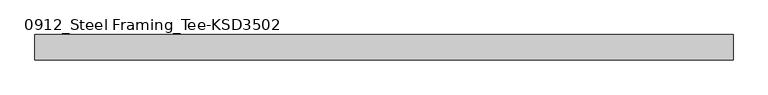
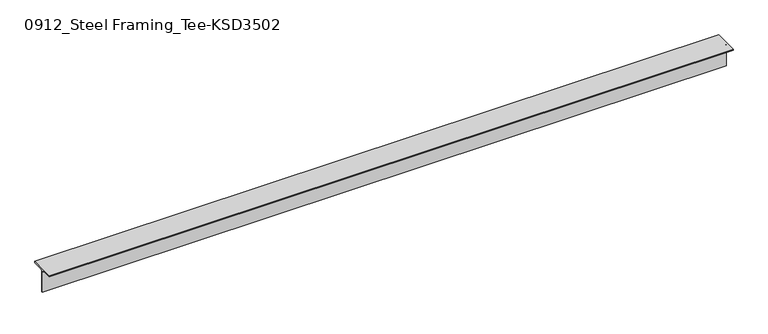
"""IFC4 building model written with IfcOpenShell, lengths in millimetres: member geometry, 0912_Steel Framing_Tee-KSD3502 : H_SB_ASB_CT-150x150x6.5x9."""

from ifc_helpers import new_model, si_unit, point, frame, frame_2d, origin, place, context, project, spatial, polyline, circle_curve, trimmed, segment, composite_curve, outline, extrude, source, transform, mapped, element, save


def member_0912_steel_framing_tee_ksd3502_90e65c15(model_context):
    return source(origin(), model_context, "Body", "SweptSolid", [
        extrude(outline(composite_curve([segment(polyline([(-75.0, 75.0), (75.0, 75.0), (75.0, 66.0), (16.25, 66.0)]), True, "CONTINUOUS"), segment(trimmed(circle_curve(frame_2d((16.25, 53.0)), 13.0), [point((16.25, 66.0))], [point((3.25, 53.0))], True, "CARTESIAN"), True, "CONTINUOUS"), segment(polyline([(3.25, 53.0), (3.25, -75.0), (-3.25, -75.0), (-3.25, 53.0)]), True, "CONTINUOUS"), segment(trimmed(circle_curve(frame_2d((-16.25, 53.0)), 13.0), [point((-3.25, 53.0))], [point((-16.25, 66.0))], True, "CARTESIAN"), True, "CONTINUOUS"), segment(polyline([(-16.25, 66.0), (-75.0, 66.0), (-75.0, 75.0)]), True, "CONTINUOUS")], self_intersect=False)), frame((-2093.8, 0.0, 0.0), z_axis=(1.0, 0.0, 0.0), x_axis=(0.0, 1.0, 0.0)), (0.0, 0.0, 1.0), 4153.3),
    ])


if __name__ == "__main__":
    model = new_model("IFC4")
    model_context = context("Model", 3, world=origin())
    ifc_project = project(units=[si_unit("LENGTHUNIT", "METRE", prefix="MILLI")], contexts=[model_context])
    site = spatial("IfcSite", under=ifc_project)
    building = spatial("IfcBuilding", under=site)
    placement = place(None, origin())
    member_0912_steel_framing_tee_ksd3502_shape = member_0912_steel_framing_tee_ksd3502_90e65c15(model_context)
    element("IfcMember", 1, ObjectType="0912_Steel Framing_Tee-KSD3502 : H_SB_ASB_CT-150x150x6.5x9", at=placement, inside=building, context=model_context, shape_type="MappedRepresentation", body=[
        mapped(member_0912_steel_framing_tee_ksd3502_shape, transform((0.0, 0.0, 0.0), x_axis=(1.0, 0.0, 0.0), y_axis=(0.0, 1.0, 0.0), z_axis=(0.0, 0.0, 1.0))),
    ])
    save(model, "model.ifc")

# Revit data of these elements
# Type "0912_Steel Framing_Tee-KSD3502 : H_SB_ASB_CT-150x150x6.5x9"
#   H_WM Code_1 = "S01AA003-00001 | Main Steel Structure Fabrication Work | Shelter/Building | Light Steel - Standard (30KG/M>Weight) | Material: (   )"
#   H_WM Code_2 = "S03AA029-00001 | Main Steel Structure Erection Work | Shelter/Building | Light Steel (30KG/M>Weight) | Material: (   )"
#   H_WM Code_3 = "S01AA010-00001 | Main Steel Structure Fabrication Work | Shelter/Building | Steel Painting/Coating | for Non-Fireproofed Steel Surface, Surface Preparation, Primer, Second & Final Coat | Material: (   )"
#   H_Q'ty Cal Type Tag = "SB-Q2"
#   Width = 15.0 cm
#   Web Thickness = 0.65 cm
#   Web Fillet = 1.3 cm
#   Section Area = 23.39 cm²
#   Perimeter = 0.60 m²/m
#   Nominal Weight = 18.40 kgf/m
#   Height = 15.0 cm
#   Flange Thickness = 0.9 cm
#   Centroid Vertical = 7.5 cm
#   Centroid Horizontal = 7.5 cm
#   Length [instance default] = 1.5000 m
#   Structural Material [instance default] = Steel, 45-345
#   Warping Constant = (empty or 0)
#   Torsional Moment of Inertia = 0
#   Section Name Key = ""
#   Plastic Modulus weak axis = 0
#   Plastic Modulus strong axis = 0
#   Moment of Inertia weak axis = 0
#   Moment of Inertia strong axis = 0
#   Elastic Modulus weak axis = 0
#   Elastic Modulus strong axis = 0
#   Bolt Spacing = 0
#   Assembly Code = ""
# Element 1 (IfcMember, "0912_Steel Framing_Tee-KSD3502 : H_SB_ASB_CT-150x150x6.5x9")
#   Structural Material = none
# Materials
#   "Steel, 45-345": class "Metal", colour RGB 189 187 185, transparency 0, Description = "Steel 345 MPa", Cost = 0
